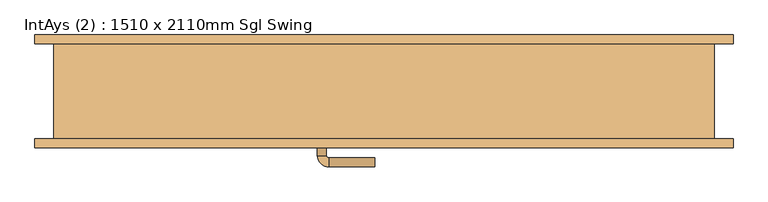
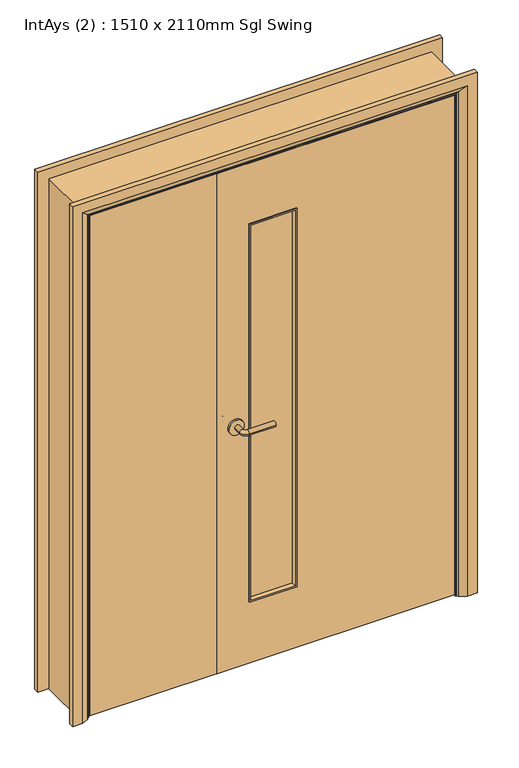
"""IFC4 building model written with IfcOpenShell, lengths in millimetres: door geometry, IntAys (2) : 1510 x 2110mm Sgl Swing."""

import ifcopenshell
import ifcopenshell.guid

model = None  # the IFC model being written
_history = None  # IfcOwnerHistory: only IFC2X3 demands one
_inside = {}  # id of a spatial element -> (the spatial element, [elements in it])
_under = {}  # id of a project, library or spatial element -> (it, [spatial elements below it])
_declared = {}  # id of a project -> (the project, [libraries it declares])
_typed = {}  # id of a type object -> (the type object, [elements of that type])
_made_of = {}  # id of a material, layer set ... -> (it, [elements and type objects made of it])


def new_model(schema):
    """Start an empty IFC model of exactly this schema.

    Asked for "IFC4X3", IfcOpenShell would pick the latest addendum, in which some entities
    have other attributes; the version numbers below select the first issue.
    IFC2X3 requires an IfcOwnerHistory on every rooted entity: one is made here for all.
    """
    global model, _history
    if schema == "IFC4X3":
        model = ifcopenshell.file(schema_version=(4, 3, 0, 0))
    else:
        model = ifcopenshell.file(schema=schema)
    _inside.clear()
    _under.clear()
    _declared.clear()
    _typed.clear()
    _made_of.clear()
    _history = None
    if model.schema == "IFC2X3":
        org = make("IfcOrganization", Name="unknown")
        user = make(
            "IfcPersonAndOrganization",
            ThePerson=make("IfcPerson", FamilyName="unknown"),
            TheOrganization=org,
        )
        app = make(
            "IfcApplication",
            ApplicationDeveloper=org,
            Version="unknown",
            ApplicationFullName="unknown",
            ApplicationIdentifier="unknown",
        )
        _history = make(
            "IfcOwnerHistory",
            OwningUser=user,
            OwningApplication=app,
            ChangeAction="ADDED",
            CreationDate=0,
        )
    return model


def make(cls, **values):
    """One entity of the class cls with the attributes given. An attribute that is None is left unset."""
    return model.create_entity(
        cls, **{name: value for name, value in values.items() if value is not None}
    )


def rooted(cls, **values):
    """An entity with a GlobalId (a new one), such as an element, a storey or a relation."""
    return make(cls, GlobalId=ifcopenshell.guid.new(), OwnerHistory=_history, **values)


def si_unit(unit_type, name, prefix=None):
    """IfcSIUnit, for example si_unit("LENGTHUNIT", "METRE", prefix="MILLI")."""
    return make("IfcSIUnit", UnitType=unit_type, Prefix=prefix, Name=name)


def assignment(units):
    """IfcUnitAssignment: the units of a project."""
    return None if units is None else make("IfcUnitAssignment", Units=units)


def point(xyz):
    """IfcCartesianPoint."""
    return None if xyz is None else make("IfcCartesianPoint", Coordinates=xyz)


def direction(xyz):
    """IfcDirection."""
    return None if xyz is None else make("IfcDirection", DirectionRatios=xyz)


def frame(location, z_axis=None, x_axis=None):
    """IfcAxis2Placement3D, a coordinate frame: its origin and axes. An axis left out is left unset."""
    return make(
        "IfcAxis2Placement3D",
        Location=point(location),
        Axis=direction(z_axis),
        RefDirection=direction(x_axis),
    )


def frame_2d(location, x_axis=None):
    """IfcAxis2Placement2D, a coordinate frame in the plane: its origin and x axis."""
    return make(
        "IfcAxis2Placement2D", Location=point(location), RefDirection=direction(x_axis)
    )


def origin():
    """The frame at (0, 0, 0) with its axes left unset."""
    return frame((0.0, 0.0, 0.0))


def place(relative_to, where):
    """IfcLocalPlacement: puts the frame where relative to a parent placement (None: the world)."""
    return make(
        "IfcLocalPlacement", PlacementRelTo=relative_to, RelativePlacement=where
    )


def context(
    kind, dimensions, precision=None, world=None, true_north=None, identifier=None
):
    """IfcGeometricRepresentationContext, for example the 3D "Model" context."""
    return make(
        "IfcGeometricRepresentationContext",
        ContextIdentifier=identifier,
        ContextType=kind,
        CoordinateSpaceDimension=dimensions,
        Precision=precision,
        WorldCoordinateSystem=world,
        TrueNorth=true_north,
    )


def project(units=None, contexts=None):
    """IfcProject with its units and contexts."""
    return rooted(
        "IfcProject",
        Name="project",
        RepresentationContexts=contexts,
        UnitsInContext=assignment(units),
    )


def spatial(cls, under=None, at=None, **own):
    """A site, building, storey or space (cls), placed at a placement, below another one or the project."""
    s = rooted(cls, ObjectPlacement=at, **own)
    if under is not None:
        _under.setdefault(under.id(), (under, []))[1].append(s)
    return s


def polyline(points):
    """IfcPolyline through the points."""
    return make("IfcPolyline", Points=[point(p) for p in points])


def circle_curve(where, radius):
    """IfcCircle in the frame where."""
    return make("IfcCircle", Position=where, Radius=radius)


def ellipse_curve(where, semi_axis1, semi_axis2):
    """IfcEllipse in the frame where."""
    return make(
        "IfcEllipse", Position=where, SemiAxis1=semi_axis1, SemiAxis2=semi_axis2
    )


def trimmed(basis, trim1, trim2, sense, master):
    """IfcTrimmedCurve: the piece of a basis curve between two trims."""
    return make(
        "IfcTrimmedCurve",
        BasisCurve=basis,
        Trim1=trim1,
        Trim2=trim2,
        SenseAgreement=sense,
        MasterRepresentation=master,
    )


def segment(curve, same_sense, transition):
    """IfcCompositeCurveSegment."""
    return make(
        "IfcCompositeCurveSegment",
        Transition=transition,
        SameSense=same_sense,
        ParentCurve=curve,
    )


def composite_curve(segments, self_intersect=None):
    """IfcCompositeCurve: segments joined end to end."""
    return make("IfcCompositeCurve", Segments=segments, SelfIntersect=self_intersect)


def outline(outer, holes=None, kind="AREA"):
    """IfcArbitraryClosedProfileDef: a profile drawn as a closed curve; with holes, ...WithVoids."""
    if holes is None:
        return make("IfcArbitraryClosedProfileDef", ProfileType=kind, OuterCurve=outer)
    return make(
        "IfcArbitraryProfileDefWithVoids",
        ProfileType=kind,
        OuterCurve=outer,
        InnerCurves=holes,
    )


def extrude(swept, where, along, depth):
    """IfcExtrudedAreaSolid: the profile swept, set in the frame where, extruded along a direction by depth."""
    return make(
        "IfcExtrudedAreaSolid",
        SweptArea=swept,
        Position=where,
        ExtrudedDirection=direction(along),
        Depth=depth,
    )


def faces_of(points, faces, orient=None, outer=None):
    """IfcFace entities. A face is a list of loops; a loop is a list of indices into points, from 0.

    orient and outer hold one flag for each loop. By default every Orientation is true, the
    first loop of a face is its IfcFaceOuterBound and the others are IfcFaceBound.
    """
    made = []
    for i, loops in enumerate(faces):
        bounds = []
        for j, loop in enumerate(loops):
            is_outer = j == 0 if outer is None else outer[i][j]
            bounds.append(
                make(
                    "IfcFaceOuterBound" if is_outer else "IfcFaceBound",
                    Bound=make("IfcPolyLoop", Polygon=[points[k] for k in loop]),
                    Orientation=True if orient is None else orient[i][j],
                )
            )
        made.append(make("IfcFace", Bounds=bounds))
    return made


def faceted_brep(points, faces, orient=None, outer=None, voids=None):
    """IfcFacetedBrep: a solid bounded by flat faces; with voids (closed shells), ...WithVoids."""
    shared = [point(p) for p in points]
    hull = make("IfcClosedShell", CfsFaces=faces_of(shared, faces, orient, outer))
    if voids is None:
        return make("IfcFacetedBrep", Outer=hull)
    return make(
        "IfcFacetedBrepWithVoids",
        Outer=hull,
        Voids=[
            make(cls, CfsFaces=faces_of(shared, fs, o, b)) for cls, fs, o, b in voids
        ],
    )


def shape(context_of_items, identifier, shape_type, items):
    """IfcShapeRepresentation: the items that make up one representation, for example the "Body"."""
    return make(
        "IfcShapeRepresentation",
        ContextOfItems=context_of_items,
        RepresentationIdentifier=identifier,
        RepresentationType=shape_type,
        Items=items,
    )


def source(mapping_origin, context_of_items, identifier, shape_type, items):
    """IfcRepresentationMap: a shape defined once, which mapped items show again and again."""
    return make(
        "IfcRepresentationMap",
        MappingOrigin=mapping_origin,
        MappedRepresentation=shape(context_of_items, identifier, shape_type, items),
    )


def transform(
    local_origin,
    x_axis=None,
    y_axis=None,
    z_axis=None,
    scale=None,
    scale2=None,
    scale3=None,
    uniform=True,
):
    """IfcCartesianTransformationOperator3D, or its non-uniform kind. x_axis, y_axis, z_axis: its Axis1, 2, 3."""
    if uniform:
        return make(
            "IfcCartesianTransformationOperator3D",
            Axis1=direction(x_axis),
            Axis2=direction(y_axis),
            LocalOrigin=point(local_origin),
            Scale=scale,
            Axis3=direction(z_axis),
        )
    return make(
        "IfcCartesianTransformationOperator3DnonUniform",
        Axis1=direction(x_axis),
        Axis2=direction(y_axis),
        LocalOrigin=point(local_origin),
        Scale=scale,
        Axis3=direction(z_axis),
        Scale2=scale2,
        Scale3=scale3,
    )


def mapped(mapping_source, mapping_target):
    """IfcMappedItem: shows the shape of a source again, moved by a transform."""
    return make(
        "IfcMappedItem", MappingSource=mapping_source, MappingTarget=mapping_target
    )


def made_of(thing, what):
    """Note that an element or type object is made of a material, layer set ...; save() writes the relation."""
    if what is not None:
        _made_of.setdefault(what.id(), (what, []))[1].append(thing)
    return thing


def element(
    cls,
    number,
    at=None,
    inside=None,
    cuts=None,
    type_object=None,
    material=None,
    context=None,
    identifier="Body",
    shape_type=None,
    held_by="IfcProductDefinitionShape",
    body=None,
    shapes=None,
    **own,
):
    """One element of the class cls, such as IfcWall. Its Tag is "e" and its number.

    at: its placement. inside: the storey or other place that contains it. cuts: it is an
    opening in that element (IfcRelVoidsElement). A single representation is given by context,
    identifier, shape_type and body (its items); several are given by shapes. held_by: the class
    of the entity that holds the representations. save() writes the other relations.
    """
    e = rooted(cls, Tag="e%d" % number, ObjectPlacement=at, **own)
    if body is not None:
        shapes = [shape(context, identifier, shape_type, body)]
    if shapes is not None:
        e.Representation = make(held_by, Representations=shapes)
    if inside is not None:
        _inside.setdefault(inside.id(), (inside, []))[1].append(e)
    if cuts is not None:
        rooted(
            "IfcRelVoidsElement", RelatingBuildingElement=cuts, RelatedOpeningElement=e
        )
    if type_object is not None:
        _typed.setdefault(type_object.id(), (type_object, []))[1].append(e)
    return made_of(e, material)


def aggregate(whole, parts):
    """IfcRelAggregates: a whole, such as a stair, and the parts it consists of."""
    return rooted("IfcRelAggregates", RelatingObject=whole, RelatedObjects=parts)


def save(model, path):
    """Write the relations noted so far, then the file.

    IfcRelAggregates (storeys below a building ...), IfcRelContainedInSpatialStructure (elements
    in a storey), IfcRelDefinesByType, IfcRelAssociatesMaterial and IfcRelDeclares: one each for
    every whole, place, type object, material and project.
    """
    for whole, parts in _under.values():
        aggregate(whole, parts)
    for where, things in _inside.values():
        rooted(
            "IfcRelContainedInSpatialStructure",
            RelatedElements=things,
            RelatingStructure=where,
        )
    for kind, things in _typed.values():
        rooted("IfcRelDefinesByType", RelatedObjects=things, RelatingType=kind)
    for what, things in _made_of.values():
        rooted("IfcRelAssociatesMaterial", RelatedObjects=things, RelatingMaterial=what)
    for by, libraries in _declared.values():
        rooted("IfcRelDeclares", RelatingContext=by, RelatedDefinitions=libraries)
    model.write(path)


def plane_surface(at):
    """IfcPlane: the flat surface through the origin of the frame at, square to its z axis."""
    return make("IfcPlane", Position=at)


def cylinder_surface(at, radius):
    """IfcCylindricalSurface: all points at the distance radius from the z axis of the frame at."""
    return make("IfcCylindricalSurface", Position=at, Radius=radius)


def revolved_surface(curve, axis_point, axis_direction):
    """IfcSurfaceOfRevolution: the curve turned about the line through axis_point along axis_direction."""
    return make(
        "IfcSurfaceOfRevolution",
        SweptCurve=make("IfcArbitraryOpenProfileDef", ProfileType="CURVE", Curve=curve),
        AxisPosition=make("IfcAxis1Placement", Location=point(axis_point), Axis=direction(axis_direction)),
    )


def advanced_brep(points, edges, surfaces, faces):
    """IfcAdvancedBrep: a solid bounded by faces that lie on surfaces and meet in shared edges.

    An edge is (start, end): straight between two places in points (the first is 0);
    or (start, end, curve); or (start, end, curve, False) where it runs against its curve.
    A face is (place in surfaces, loops), or (place, loops, False) where it looks against
    its surface's normal. A loop lists edges by number (the first is 1), with a minus sign
    where the edge is run from its end to its start. The first loop is the outer one.
    """
    corners = [point(p) for p in points]
    vertices = [make("IfcVertexPoint", VertexGeometry=c) for c in corners]
    made = []
    for start, end, *more in edges:
        made.append(
            make(
                "IfcEdgeCurve",
                EdgeStart=vertices[start],
                EdgeEnd=vertices[end],
                EdgeGeometry=more[0] if more else make("IfcPolyline", Points=[corners[start], corners[end]]),
                SameSense=more[1] if len(more) > 1 else True,
            )
        )
    hull = []
    for where, loops, *sense in faces:
        bounds = []
        for j, loop in enumerate(loops):
            ring = [make("IfcOrientedEdge", EdgeElement=made[abs(k) - 1], Orientation=k > 0) for k in loop]
            bounds.append(
                make(
                    "IfcFaceOuterBound" if j == 0 else "IfcFaceBound",
                    Bound=make("IfcEdgeLoop", EdgeList=ring),
                    Orientation=True,
                )
            )
        hull.append(make("IfcAdvancedFace", Bounds=bounds, FaceSurface=surfaces[where], SameSense=sense[0] if sense else True))
    return make("IfcAdvancedBrep", Outer=make("IfcClosedShell", CfsFaces=hull))


def intays_2_1510_x_2110mm_sgl_swing_dce9c54a(model_context):
    return source(origin(), model_context, "Body", "SolidModel", [
        advanced_brep(
        [(88.5, -67.5, 1000.0), (108.5, -67.5, 1000.0), (88.5, -37.5, 1000.0), (108.5, -37.5, 1000.0), (113.5, -32.5, 1000.0), (113.5, -12.5, 1000.0), (218.5, -12.5, 1000.0), (218.5, -32.5, 1000.0)],
        [
            (0, 1, circle_curve(frame((98.5, -67.5, 1000.0), z_axis=(0.0, -1.0, 0.0), x_axis=(1.0, 0.0, 0.0)), 10.0)),
            (1, 0, circle_curve(frame((98.5, -67.5, 1000.0), z_axis=(0.0, -1.0, 0.0), x_axis=(1.0, 0.0, 0.0)), 10.0)),
            (0, 2),
            (2, 3, circle_curve(frame((98.5, -37.5, 1000.0), z_axis=(0.0, -1.0, 0.0), x_axis=(1.0, 0.0, 0.0)), 10.0)),
            (3, 1),
            (3, 2, circle_curve(frame((98.5, -37.5, 1000.0), z_axis=(0.0, -1.0, 0.0), x_axis=(1.0, 0.0, 0.0)), 10.0)),
            (4, 3, circle_curve(frame((113.5, -37.5, 1000.0), z_axis=(0.0, 0.0, 1.0), x_axis=(-1.0, 0.0, 0.0)), 5.0)),
            (2, 5, circle_curve(frame((113.5, -37.5, 1000.0), z_axis=(0.0, 0.0, -1.0), x_axis=(-1.0, 0.0, 0.0)), 25.0)),
            (5, 4, circle_curve(frame((113.5, -22.5, 1000.0), z_axis=(-1.0, 0.0, 0.0), x_axis=(0.0, -1.0, 0.0)), 10.0)),
            (4, 5, circle_curve(frame((113.5, -22.5, 1000.0), z_axis=(-1.0, 0.0, 0.0), x_axis=(0.0, -1.0, 0.0)), 10.0)),
            (6, 7, circle_curve(frame((218.5, -22.5, 1000.0), z_axis=(1.0, 0.0, 0.0), x_axis=(0.0, -1.0, 0.0)), 10.0)),
            (7, 6, circle_curve(frame((218.5, -22.5, 1000.0), z_axis=(1.0, 0.0, 0.0), x_axis=(0.0, -1.0, 0.0)), 10.0)),
            (5, 6),
            (7, 4),
        ],
        [
            plane_surface(frame((98.5, -67.5, 1000.0), z_axis=(0.0, -1.0, 0.0), x_axis=(0.0, 0.0, 1.0))),
            cylinder_surface(frame((98.5, -67.5, 1000.0), z_axis=(0.0, -1.0, 0.0), x_axis=(1.0, 0.0, 0.0)), 10.0),
            revolved_surface(trimmed(ellipse_curve(frame((98.5, -37.5, 1000.0), z_axis=(0.0, -1.0, 0.0), x_axis=(1.0, 0.0, 0.0)), 10.0, 10.0), [point((88.5, -37.5, 1000.0))], [point((108.5, -37.5, 1000.0))], True, "CARTESIAN"), (113.5, -37.5, 1000.0), (0.0, 0.0, -1.0)),
            revolved_surface(trimmed(ellipse_curve(frame((98.5, -37.5, 1000.0), z_axis=(0.0, -1.0, 0.0), x_axis=(1.0, 0.0, 0.0)), 10.0, 10.0), [point((108.5, -37.5, 1000.0))], [point((88.5, -37.5, 1000.0))], True, "CARTESIAN"), (113.5, -37.5, 1000.0), (0.0, 0.0, -1.0)),
            plane_surface(frame((218.5, -22.5, 1000.0), z_axis=(1.0, 0.0, 0.0), x_axis=(0.0, 0.0, 1.0))),
            cylinder_surface(frame((113.5, -22.5, 1000.0), z_axis=(-1.0, 0.0, 0.0), x_axis=(0.0, -1.0, 0.0)), 10.0),
        ],
        [
            (0, [[1, 2]]),
            (1, [[-1, 3, 4, 5]]),
            (1, [[-2, -5, 6, -3]]),
            (2, [[7, -4, 8, 9]]),
            (3, [[-8, -6, -7, 10]]),
            (4, [[11, 12]]),
            (5, [[-9, 13, -12, 14]]),
            (5, [[-10, -14, -11, -13]]),
        ],
    ),
        extrude(outline(composite_curve([segment(trimmed(circle_curve(frame_2d((1000.0, 96.0)), 30.0), [point((1000.0, 66.0))], [point((1000.0, 126.0))], False, "CARTESIAN"), True, "CONTINUOUS"), segment(trimmed(circle_curve(frame_2d((1000.0, 96.0)), 30.0), [point((1000.0, 126.0))], [point((1000.0, 66.0))], False, "CARTESIAN"), True, "CONTINUOUS")], self_intersect=False)), frame((0.0, -75.5, 0.0), z_axis=(0.0, 1.0, 0.0), x_axis=(0.0, 0.0, 1.0)), (0.0, 0.0, 1.0), 8.0),
        advanced_brep(
        [(88.5, -115.5, 1000.0), (108.5, -115.5, 1000.0), (108.5, -145.5, 1000.0), (88.5, -145.5, 1000.0), (113.5, -150.5, 1000.0), (113.5, -170.5, 1000.0), (218.5, -170.5, 1000.0), (218.5, -150.5, 1000.0)],
        [
            (0, 1, circle_curve(frame((98.5, -115.5, 1000.0), z_axis=(0.0, 1.0, 0.0), x_axis=(1.0, 0.0, 0.0)), 10.0)),
            (1, 0, circle_curve(frame((98.5, -115.5, 1000.0), z_axis=(0.0, 1.0, 0.0), x_axis=(1.0, 0.0, 0.0)), 10.0)),
            (1, 2),
            (2, 3, circle_curve(frame((98.5, -145.5, 1000.0), z_axis=(0.0, 1.0, 0.0), x_axis=(1.0, 0.0, 0.0)), 10.0)),
            (3, 0),
            (3, 2, circle_curve(frame((98.5, -145.5, 1000.0), z_axis=(0.0, 1.0, 0.0), x_axis=(1.0, 0.0, 0.0)), 10.0)),
            (4, 5, circle_curve(frame((113.5, -160.5, 1000.0), z_axis=(-1.0, 0.0, 0.0), x_axis=(0.0, 1.0, 0.0)), 10.0)),
            (5, 3, circle_curve(frame((113.5, -145.5, 1000.0), z_axis=(0.0, 0.0, -1.0), x_axis=(-1.0, 0.0, 0.0)), 25.0)),
            (2, 4, circle_curve(frame((113.5, -145.5, 1000.0), z_axis=(0.0, 0.0, 1.0), x_axis=(-1.0, 0.0, 0.0)), 5.0)),
            (5, 4, circle_curve(frame((113.5, -160.5, 1000.0), z_axis=(-1.0, 0.0, 0.0), x_axis=(0.0, 1.0, 0.0)), 10.0)),
            (6, 7, circle_curve(frame((218.5, -160.5, 1000.0), z_axis=(1.0, 0.0, 0.0), x_axis=(0.0, 1.0, 0.0)), 10.0)),
            (7, 6, circle_curve(frame((218.5, -160.5, 1000.0), z_axis=(1.0, 0.0, 0.0), x_axis=(0.0, 1.0, 0.0)), 10.0)),
            (4, 7),
            (6, 5),
        ],
        [
            plane_surface(frame((98.5, -115.5, 1000.0), z_axis=(0.0, 1.0, 0.0), x_axis=(0.0, 0.0, 1.0))),
            cylinder_surface(frame((98.5, -115.5, 1000.0), z_axis=(0.0, 1.0, 0.0), x_axis=(1.0, 0.0, 0.0)), 10.0),
            revolved_surface(trimmed(ellipse_curve(frame((98.5, -145.5, 1000.0), z_axis=(0.0, -1.0, 0.0), x_axis=(1.0, 0.0, 0.0)), 10.0, 10.0), [point((88.5, -145.5, 1000.0))], [point((108.5, -145.5, 1000.0))], True, "CARTESIAN"), (113.5, -145.5, 1000.0), (0.0, 0.0, -1.0)),
            revolved_surface(trimmed(ellipse_curve(frame((98.5, -145.5, 1000.0), z_axis=(0.0, -1.0, 0.0), x_axis=(1.0, 0.0, 0.0)), 10.0, 10.0), [point((108.5, -145.5, 1000.0))], [point((88.5, -145.5, 1000.0))], True, "CARTESIAN"), (113.5, -145.5, 1000.0), (0.0, 0.0, -1.0)),
            plane_surface(frame((218.5, -160.5, 1000.0), z_axis=(1.0, 0.0, 0.0), x_axis=(0.0, 0.0, 1.0))),
            cylinder_surface(frame((113.5, -160.5, 1000.0), z_axis=(-1.0, 0.0, 0.0), x_axis=(0.0, 1.0, 0.0)), 10.0),
        ],
        [
            (0, [[1, 2]]),
            (1, [[3, 4, 5, -2]]),
            (1, [[-5, 6, -3, -1]]),
            (2, [[7, 8, -4, 9]]),
            (3, [[10, -9, -6, -8]]),
            (4, [[11, 12]]),
            (5, [[13, -11, 14, -7]]),
            (5, [[-14, -12, -13, -10]]),
        ],
    ),
        extrude(outline(composite_curve([segment(trimmed(circle_curve(frame_2d((1000.0, 96.0)), 30.0), [point((1000.0, 66.0))], [point((1000.0, 126.0))], False, "CARTESIAN"), True, "CONTINUOUS"), segment(trimmed(circle_curve(frame_2d((1000.0, 96.0)), 30.0), [point((1000.0, 126.0))], [point((1000.0, 66.0))], False, "CARTESIAN"), True, "CONTINUOUS")], self_intersect=False)), frame((0.0, -115.5, 0.0), z_axis=(0.0, 1.0, 0.0), x_axis=(0.0, 0.0, 1.0)), (0.0, 0.0, 1.0), 8.0),
        extrude(outline(polyline([(2102.0, -508.0), (0.0, -508.0), (0.0, -476.0), (2070.0, -476.0), (2070.0, 954.0), (0.0, 954.0), (0.0, 986.0), (2102.0, 986.0), (2102.0, -508.0)])), frame((0.0, -107.5, 0.0), z_axis=(0.0, 1.0, 0.0), x_axis=(0.0, 0.0, 1.0)), (0.0, 0.0, 1.0), 215.0),
        advanced_brep(
        [(-551.0, 127.5, 0.0), (-511.0, 127.5, 0.0), (-485.0, 113.5, 0.0), (-481.0, 107.5, 0.0), (-551.0, 107.5, 0.0), (-551.0, 107.5, 2145.0), (-551.0, 127.5, 2145.0), (-481.0, 107.5, 2075.0), (959.0, 107.5, 2075.0), (959.0, 107.5, 0.0), (1029.0, 107.5, 0.0), (1029.0, 107.5, 2145.0), (-485.0, 113.5, 2079.0), (-511.0, 127.5, 2105.0), (1029.0, 127.5, 2145.0), (1029.0, 127.5, 0.0), (989.0, 127.5, 0.0), (989.0, 127.5, 2105.0), (963.0, 113.5, 0.0), (963.0, 113.5, 2079.0)],
        [
            (0, 1),
            (1, 2),
            (2, 3, circle_curve(frame((-489.0, 106.5, 0.0), z_axis=(0.0, 0.0, -1.0), x_axis=(-1.0, 0.0, 0.0)), 8.0622577)),
            (3, 4),
            (4, 0),
            (4, 5),
            (5, 6),
            (6, 0),
            (3, 7),
            (7, 8),
            (8, 9),
            (9, 10),
            (10, 11),
            (11, 5),
            (2, 12),
            (12, 7, ellipse_curve(frame((-489.0, 106.5, 2083.0), z_axis=(-0.7071067811865475, 0.0, -0.7071067811865475), x_axis=(0.7071067811865474, 0.0, -0.7071067811865476)), 11.4017543, 8.0622577)),
            (1, 13),
            (13, 12),
            (6, 14),
            (14, 15),
            (15, 16),
            (16, 17),
            (17, 13),
            (10, 15),
            (14, 11),
            (9, 18, circle_curve(frame((967.0, 106.5, 0.0), z_axis=(0.0, 0.0, -1.0), x_axis=(1.0, 0.0, 0.0)), 8.0622577)),
            (18, 16),
            (19, 18),
            (8, 19, ellipse_curve(frame((967.0, 106.5, 2083.0), z_axis=(0.7071067811865475, 0.0, -0.7071067811865475), x_axis=(0.7071067811865474, 0.0, 0.7071067811865476)), 11.4017543, 8.0622577)),
            (19, 17),
            (12, 19),
        ],
        [
            plane_surface(frame((-481.0, 107.5, 0.0), z_axis=(0.0, 0.0, -1.0), x_axis=(0.0, 1.0, 0.0))),
            plane_surface(frame((-551.0, 127.5, 0.0), z_axis=(-1.0, 0.0, 0.0), x_axis=(0.0, 0.0, 1.0))),
            plane_surface(frame((-551.0, 107.5, 0.0), z_axis=(0.0, -1.0, 0.0), x_axis=(0.0, 0.0, 1.0))),
            cylinder_surface(frame((-489.0, 106.5, 0.0), z_axis=(0.0, 0.0, -1.0), x_axis=(-1.0, 0.0, 0.0)), 8.0622577),
            plane_surface(frame((-485.0, 113.5, 0.0), z_axis=(0.4740998230350183, 0.8804710999221749, 0.0), x_axis=(0.0, 0.0, 1.0))),
            plane_surface(frame((-511.0, 127.5, 0.0), z_axis=(0.0, 1.0, 0.0), x_axis=(0.0, 0.0, 1.0))),
            plane_surface(frame((1029.0, 127.5, 2145.0), z_axis=(1.0, 0.0, 0.0), x_axis=(0.0, 0.0, -1.0))),
            plane_surface(frame((959.0, 107.5, 0.0), z_axis=(0.0, 0.0, -1.0), x_axis=(0.0, 1.0, 0.0))),
            cylinder_surface(frame((967.0, 106.5, 2075.0), z_axis=(0.0, 0.0, 1.0), x_axis=(1.0, 0.0, 0.0)), 8.0622577),
            plane_surface(frame((963.0, 113.5, 2079.0), z_axis=(-0.4740998230350183, 0.8804710999221749, 0.0), x_axis=(0.0, 0.0, -1.0))),
            plane_surface(frame((-551.0, 127.5, 2145.0), z_axis=(0.0, 0.0, 1.0), x_axis=(1.0, 0.0, 0.0))),
            cylinder_surface(frame((-481.0, 106.5, 2083.0), z_axis=(-1.0, 0.0, 0.0), x_axis=(0.0, 0.0, 1.0)), 8.0622577),
            plane_surface(frame((-485.0, 113.5, 2079.0), z_axis=(0.0, 0.8804710999221749, -0.4740998230350183), x_axis=(1.0, 0.0, 0.0))),
        ],
        [
            (0, [[1, 2, 3, 4, 5]]),
            (1, [[6, 7, 8, -5]]),
            (2, [[9, 10, 11, 12, 13, 14, -6, -4]]),
            (3, [[15, 16, -9, -3]]),
            (4, [[17, 18, -15, -2]]),
            (5, [[-8, 19, 20, 21, 22, 23, -17, -1]]),
            (6, [[-13, 24, -20, 25]]),
            (7, [[-24, -12, 26, 27, -21]]),
            (8, [[28, -26, -11, 29]]),
            (9, [[-22, -27, -28, 30]]),
            (10, [[-14, -25, -19, -7]]),
            (11, [[31, -29, -10, -16]]),
            (12, [[-23, -30, -31, -18]]),
        ],
    ),
        advanced_brep(
        [(1029.0, -127.5, 0.0), (989.0, -127.5, 0.0), (963.0, -113.5, 0.0), (959.0, -107.5, 0.0), (1029.0, -107.5, 0.0), (1029.0, -107.5, 2145.0), (1029.0, -127.5, 2145.0), (959.0, -107.5, 2075.0), (-481.0, -107.5, 2075.0), (-481.0, -107.5, 0.0), (-551.0, -107.5, 0.0), (-551.0, -107.5, 2145.0), (963.0, -113.5, 2079.0), (989.0, -127.5, 2105.0), (-551.0, -127.5, 2145.0), (-551.0, -127.5, 0.0), (-511.0, -127.5, 0.0), (-511.0, -127.5, 2105.0), (-485.0, -113.5, 0.0), (-485.0, -113.5, 2079.0)],
        [
            (0, 1),
            (1, 2),
            (2, 3, circle_curve(frame((967.0, -106.5, 0.0), z_axis=(0.0, 0.0, -1.0), x_axis=(1.0, 0.0, 0.0)), 8.0622577)),
            (3, 4),
            (4, 0),
            (4, 5),
            (5, 6),
            (6, 0),
            (3, 7),
            (7, 8),
            (8, 9),
            (9, 10),
            (10, 11),
            (11, 5),
            (2, 12),
            (12, 7, ellipse_curve(frame((967.0, -106.5, 2083.0), z_axis=(0.7071067811865475, 0.0, -0.7071067811865475), x_axis=(-0.7071067811865474, 0.0, -0.7071067811865476)), 11.4017543, 8.0622577)),
            (1, 13),
            (13, 12),
            (6, 14),
            (14, 15),
            (15, 16),
            (16, 17),
            (17, 13),
            (10, 15),
            (14, 11),
            (9, 18, circle_curve(frame((-489.0, -106.5, 0.0), z_axis=(0.0, 0.0, -1.0), x_axis=(-1.0, 0.0, 0.0)), 8.0622577)),
            (18, 16),
            (19, 18),
            (8, 19, ellipse_curve(frame((-489.0, -106.5, 2083.0), z_axis=(-0.7071067811865475, 0.0, -0.7071067811865475), x_axis=(-0.7071067811865474, 0.0, 0.7071067811865476)), 11.4017543, 8.0622577)),
            (19, 17),
            (12, 19),
        ],
        [
            plane_surface(frame((959.0, -107.5, 0.0), z_axis=(0.0, 0.0, -1.0), x_axis=(0.0, 1.0, 0.0))),
            plane_surface(frame((1029.0, -127.5, 0.0), z_axis=(1.0, 0.0, 0.0), x_axis=(0.0, 0.0, 1.0))),
            plane_surface(frame((1029.0, -107.5, 0.0), z_axis=(0.0, 1.0, 0.0), x_axis=(0.0, 0.0, 1.0))),
            cylinder_surface(frame((967.0, -106.5, 0.0), z_axis=(0.0, 0.0, -1.0), x_axis=(1.0, 0.0, 0.0)), 8.0622577),
            plane_surface(frame((963.0, -113.5, 0.0), z_axis=(-0.4740998230350126, -0.8804710999221779, 0.0), x_axis=(0.0, 0.0, 1.0))),
            plane_surface(frame((989.0, -127.5, 0.0), z_axis=(0.0, -1.0, 0.0), x_axis=(0.0, 0.0, 1.0))),
            plane_surface(frame((-551.0, -127.5, 2145.0), z_axis=(-1.0, 0.0, 0.0), x_axis=(0.0, 0.0, -1.0))),
            plane_surface(frame((-481.0, -107.5, 0.0), z_axis=(0.0, 0.0, -1.0), x_axis=(0.0, 1.0, 0.0))),
            cylinder_surface(frame((-489.0, -106.5, 2075.0), z_axis=(0.0, 0.0, 1.0), x_axis=(-1.0, 0.0, 0.0)), 8.0622577),
            plane_surface(frame((-485.0, -113.5, 2079.0), z_axis=(0.4740998230350183, -0.8804710999221749, 0.0), x_axis=(0.0, 0.0, -1.0))),
            plane_surface(frame((1029.0, -127.5, 2145.0), z_axis=(0.0, 0.0, 1.0), x_axis=(-1.0, 0.0, 0.0))),
            cylinder_surface(frame((959.0, -106.5, 2083.0), z_axis=(1.0, 0.0, 0.0), x_axis=(0.0, 0.0, 1.0)), 8.0622577),
            plane_surface(frame((963.0, -113.5, 2079.0), z_axis=(0.0, -0.8804710999221763, -0.4740998230350154), x_axis=(-1.0, 0.0, 0.0))),
        ],
        [
            (0, [[1, 2, 3, 4, 5]]),
            (1, [[6, 7, 8, -5]]),
            (2, [[9, 10, 11, 12, 13, 14, -6, -4]]),
            (3, [[15, 16, -9, -3]]),
            (4, [[17, 18, -15, -2]]),
            (5, [[-8, 19, 20, 21, 22, 23, -17, -1]]),
            (6, [[-13, 24, -20, 25]]),
            (7, [[-24, -12, 26, 27, -21]]),
            (8, [[28, -26, -11, 29]]),
            (9, [[-22, -27, -28, 30]]),
            (10, [[-14, -25, -19, -7]]),
            (11, [[31, -29, -10, -16]]),
            (12, [[-23, -30, -31, -18]]),
        ],
    ),
        faceted_brep([(-457.0, -72.5, 0.0), (-476.0, -72.5, 0.0), (-476.0, -40.5, 0.0), (-457.0, -40.5, 0.0), (-457.0, -40.5, 2051.0), (-457.0, -72.5, 2051.0), (-476.0, -40.5, 2070.0), (-476.0, -72.5, 2070.0), (935.0, -72.5, 0.0), (935.0, -40.5, 0.0), (954.0, -40.5, 0.0), (954.0, -72.5, 0.0), (935.0, -72.5, 2051.0), (954.0, -72.5, 2070.0), (954.0, -40.5, 2070.0), (935.0, -40.5, 2051.0)], [[[0, 1, 2, 3]], [[3, 4, 5, 0]], [[2, 6, 4, 3]], [[1, 7, 6, 2]], [[0, 5, 7, 1]], [[8, 9, 10, 11]], [[12, 8, 11, 13]], [[13, 11, 10, 14]], [[14, 10, 9, 15]], [[15, 9, 8, 12]], [[4, 15, 12, 5]], [[6, 14, 15, 4]], [[7, 13, 14, 6]], [[5, 12, 13, 7]]]),
        extrude(outline(polyline([(335.0, -85.5), (335.0, -97.5), (150.0, -97.5), (150.0, -85.5), (335.0, -85.5)])), frame((0.0, 0.0, 257.0), z_axis=(0.0, 0.0, 1.0), x_axis=(1.0, 0.0, 0.0)), (0.0, 0.0, 1.0), 1560.0),
        extrude(outline(polyline([(22.0, -75.5), (22.0, -107.5), (-473.0, -107.5), (-473.0, -75.5), (22.0, -75.5)])), frame((0.0, 0.0, 5.753223), z_axis=(0.0, 0.0, 1.0), x_axis=(1.0, 0.0, 0.0)), (0.0, 0.0, 1.0), 2061.246777),
        extrude(outline(polyline([(5.753223, 951.0), (2067.0, 951.0), (2067.0, 25.0), (5.753223, 25.0), (5.753223, 951.0)]), holes=[polyline([(1817.0, 150.0), (1817.0, 335.0), (257.0, 335.0), (257.0, 150.0), (1817.0, 150.0)])]), frame((0.0, -107.5, 0.0), z_axis=(0.0, 1.0, 0.0), x_axis=(0.0, 0.0, 1.0)), (0.0, 0.0, 1.0), 32.0),
        faceted_brep([(335.0, -72.5, 257.0), (335.0, -72.5, 1817.0), (335.0, -85.5, 1817.0), (335.0, -85.5, 257.0), (323.0, -85.5, 269.0), (323.0, -85.5, 1805.0), (329.0, -72.5, 1811.0), (329.0, -72.5, 263.0), (150.0, -72.5, 1817.0), (150.0, -85.5, 1817.0), (162.0, -85.5, 1805.0), (156.0, -72.5, 1811.0), (150.0, -72.5, 257.0), (150.0, -85.5, 257.0), (162.0, -85.5, 269.0), (156.0, -72.5, 263.0)], [[[0, 1, 2, 3]], [[4, 5, 6, 7]], [[1, 8, 9, 2]], [[5, 10, 11, 6]], [[8, 12, 13, 9]], [[10, 14, 15, 11]], [[3, 2, 9, 13], [5, 4, 14, 10]], [[12, 0, 3, 13]], [[1, 0, 12, 8], [7, 6, 11, 15]], [[14, 4, 7, 15]]]),
        faceted_brep([(150.0, -110.5, 257.0), (150.0, -110.5, 1817.0), (150.0, -97.5, 1817.0), (150.0, -97.5, 257.0), (162.0, -97.5, 269.0), (162.0, -97.5, 1805.0), (156.0, -110.5, 1811.0), (156.0, -110.5, 263.0), (335.0, -110.5, 1817.0), (335.0, -97.5, 1817.0), (323.0, -97.5, 1805.0), (329.0, -110.5, 1811.0), (335.0, -110.5, 257.0), (335.0, -97.5, 257.0), (323.0, -97.5, 269.0), (329.0, -110.5, 263.0)], [[[0, 1, 2, 3]], [[4, 5, 6, 7]], [[1, 8, 9, 2]], [[5, 10, 11, 6]], [[8, 12, 13, 9]], [[10, 14, 15, 11]], [[3, 2, 9, 13], [5, 4, 14, 10]], [[12, 0, 3, 13]], [[1, 0, 12, 8], [7, 6, 11, 15]], [[14, 4, 7, 15]]]),
    ])


if __name__ == "__main__":
    model = new_model("IFC4")
    model_context = context("Model", 3, world=origin())
    ifc_project = project(units=[si_unit("LENGTHUNIT", "METRE", prefix="MILLI")], contexts=[model_context])
    site = spatial("IfcSite", under=ifc_project)
    building = spatial("IfcBuilding", under=site)
    placement = place(None, origin())
    intays_2_1510_x_2110mm_sgl_swing_shape = intays_2_1510_x_2110mm_sgl_swing_dce9c54a(model_context)
    element("IfcDoor", 1, ObjectType="IntAys (2) : 1510 x 2110mm Sgl Swing", at=placement, inside=building, context=model_context, shape_type="MappedRepresentation", body=[
        mapped(intays_2_1510_x_2110mm_sgl_swing_shape, transform((0.0, 0.0, 0.0), x_axis=(1.0, 0.0, 0.0), y_axis=(0.0, 1.0, 0.0), z_axis=(0.0, 0.0, 1.0))),
    ])
    save(model, "model.ifc")

# Revit data of these elements
# Type "IntAys (2) : 1510 x 2110mm Sgl Swing"
#   Type Mark = "46"
#   Type Comments = "Internal Asymmetric"
#   Operation = "DoubleDoorSingleSwing"
#   Construction Type Id = "SGL"
#   Keynote = "L20"
#   Description = "Internal Asymmetric Door"
#   Analytic Construction = "Large single-glazed windows"
#   Visual Light Transmittance = 0.9
#   VisionPanel Width = 185 mm
#   Thickness = 32 mm
#   Stop Thickness = 19 mm
#   Stop Depth = 32 mm
#   Stile Top Rail = 250 mm
#   Stile Shutting = 125 mm
#   Stile Bottom Rail = 250 mm
#   Solar Heat Gain Coefficient = 0.86
#   Secondary Panel Width = 495 mm
#   Rough Width = 1510 mm
#   Rough Height = 2110 mm
#   Main Panel Width = 926 mm
#   Heat Transfer Coefficient (U) = 5.5617 W/(m²·K)
#   Handle Z Distance = 1000 mm
#   Handle X Distance = 75 mm
#   Handle Length = 350 mm
#   Frame Thickness = 32 mm
#   Door Panel Width = 926 mm
#   Door Panel Thickness = 32 mm
#   Height = 2110 mm
#   Door Panel Offset = 0 mm
#   Structural Tolerance = 8 mm
#   Tolerance = 3 mm
#   UnderCut = 7 mm
#   Width = 1510 mm
#   Door Panel Height = 2060 mm
#   Architrave Setback = 5 mm
#   Vis - Swing Single = yes
#   Vis - Swing Opposing = no
#   Vis - Swing Double = no
#   Vis - Stops = yes
#   Vis - Ironmongery = yes
#   Define Thermal Properties by = 1
#   Material Ironmongery = Door - Handle
#   Material Glass = Door - Glazing
#   Material Frame = Door - Frame/Mullion
#   Material Door = Door - Panel
#   Material Beading = Door - Panel
#   Material Architrave = Door - Architrave
#   Handle Style = element 261135
#   Function = (empty or 0)
#   Wall Closure = (empty or 0)
# Element 1 (IfcDoor, "IntAys (2) : 1510 x 2110mm Sgl Swing")
#   Materials on its faces: "Door - Panel", "Door - Architrave", "Door - Handle", "Door - Frame/Mullion", "Door - Glazing"
# Materials
#   "Door - Handle": class "Miscellaneous", colour RGB 0 0 0, transparency 0, Keynote = "P21"
#   "Door - Glazing": class "Miscellaneous", colour RGB 0 0 255, transparency 0.75
#   "Door - Frame/Mullion": class "Wood", colour RGB 212 179 113, transparency 0, Keynote = "L20"
#   "Door - Panel": class "Wood", colour RGB 210 159 95, transparency 0, Keynote = "L20"
#   "Door - Architrave": class "Wood", colour RGB 154 90 5, transparency 0, Keynote = "P20"
